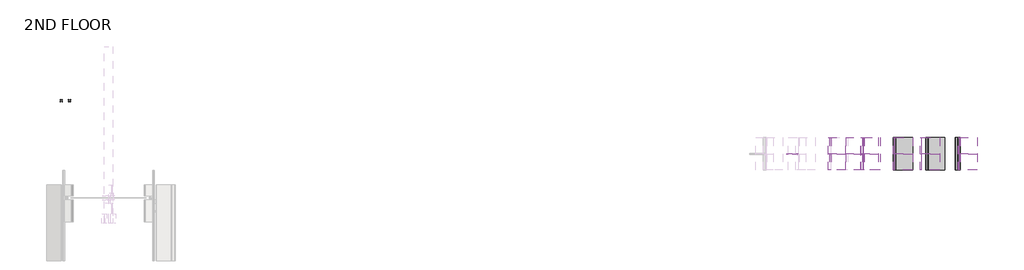
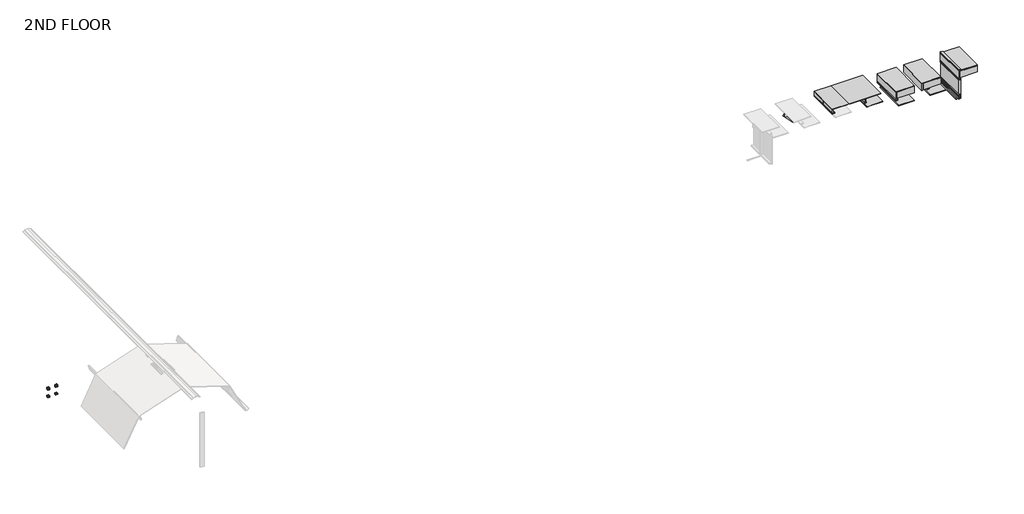
# One storey, part 2 of 2: 61 proxies.
# Revit data of these elements (continued)
# Elements 46, 47, 48, 49, 50, 51, 52, 53 (IfcBuildingElementProxy, "Lag Bolt : 1/2\" X 1 1/2\"") (continued)
#   Thickness_of_Substrate = 0' - 0 143/256"
#   Nut_Visibility = yes
#   Bolt Material (Size) = THRU-BOLT OR LAG BOLT
#   Phase Created = 1st Phase
#   Materials on its faces: "THRU-BOLT OR LAG BOLT"
# Elements 54, 55, 56, 57, 58, 59, 60, 61 (IfcBuildingElementProxy, "Lag Bolt : 1/2\" x 2 1/2\"")
#   Thickness_of_Substrate = 0' - 2 15/256"
#   Nut_Visibility = yes
#   Bolt Material (Size) = THRU-BOLT OR LAG BOLT
#   Phase Created = 1st Phase
#   Materials on its faces: "THRU-BOLT OR LAG BOLT"
# Materials
#   "1/2\" X 5\" LAG BOLT (THRU BOLT IF PLATE ON OPP. SIDE OF STRUCT MEMBER)": class "Generic", colour RGB 120 120 120, transparency 0, Cost = 0
#   "STRUCTURAL BOLTS (PAINT TO MATCH STEEL FINISH)": class "Generic", colour RGB 120 120 120, transparency 0, Cost = 0
#   "2X BLOCKING - LOCATED AT GRAB BARS, WALL HUNG CABINETS, ETC.)": class "Wood", colour RGB 234 198 147, transparency 0, Description = "Pinus Echinata", Cost = 0
#   "EXISTING GIRT": class "Metal", colour RGB 199 199 199, transparency 0, Description = "Carbon steel", Cost = 0
#   "2X WOOD HEADER ATTACHED TO EXISTING JOIST": class "Wood", colour RGB 234 198 147, transparency 0, Description = "Pinus Echinata", Cost = 0
#   "WOOD BLOCKING - SIZE AS NECESSARY": class "Wood", colour RGB 234 198 147, transparency 0, Description = "Pinus Echinata", Cost = 0
#   "(S) SOUND BATT. INSULATION (THICKNESS TO MATCH WALL DEPTH)": class "Unassigned", colour RGB 255 255 255, transparency 0, Cost = 0
#   "DOUBLE 2X WOOD TOP PLATE": class "Wood", colour RGB 234 198 147, transparency 0, Description = "Pinus Echinata", Cost = 0
#   "3/4\" CDX PLYWOOD": class "Unassigned", colour RGB 196 177 123, transparency 0, Cost = 0
#   "WOOD JOIST AS SPECIFIED": class "Wood", colour RGB 234 198 147, transparency 0, Description = "Pinus Echinata", Cost = 0
#   "RIM BOARD - SIZE TO MATCH JOIST DEPTH": class "Wood", colour RGB 234 198 147, transparency 0, Description = "Pinus Echinata", Cost = 0
#   "SOUND BATT. INSULATION": class "Unassigned", colour RGB 255 255 255, transparency 0, Cost = 0
#   "SET IN BED OF SEALANT": class "Unassigned", colour RGB 58 208 21, transparency 0, Cost = 0
#   "CEILING TRACK AS SCHEDULED": class "Unassigned", colour RGB 210 209 208, transparency 0, Keynote = "M05121300.02", Cost = 0
#   "ATTACH GYPSUM BOARD TO STUDS AND NOT TO TOP TRACK": class "Generic", colour RGB 48 48 48, transparency 0, Cost = 0
#   "EXISTING RIM BOARD OR JOIST": class "Wood", colour RGB 234 198 147, transparency 0, Description = "Pinus Echinata", Cost = 0
#   "EXISTING SUBSTRATE": class "Unassigned", colour RGB 196 177 123, transparency 0, Cost = 0
#   "DIAGONAL BRACING AS REQUIRED": class "Wood", colour RGB 234 198 147, transparency 0, Description = "Pinus Echinata", Cost = 0
#   "SUBSTRATE AS SCHEDULED": class "Unassigned", colour RGB 196 177 123, transparency 0, Cost = 0
#   "METAL RUNNER CHANNEL; FASTEN @ 24\" O.C.": class "Unassigned", colour RGB 210 209 208, transparency 0, Keynote = "M05121300.02", Cost = 0
#   "CEILING AS SCHEDULED": class "Generic", colour RGB 255 255 255, transparency 0, Cost = 0
#   "2X12 LEDGER WITH HILTI 3/8* DIAMETER HLC SLEEVE ANCHOR @ 8” OC.": class "Wood", colour RGB 234 198 147, transparency 0, Description = "Pinus Echinata", Cost = 0
#   "THRU-BOLT OR LAG BOLT": class "Generic", colour RGB 120 120 120, transparency 0, Cost = 0
